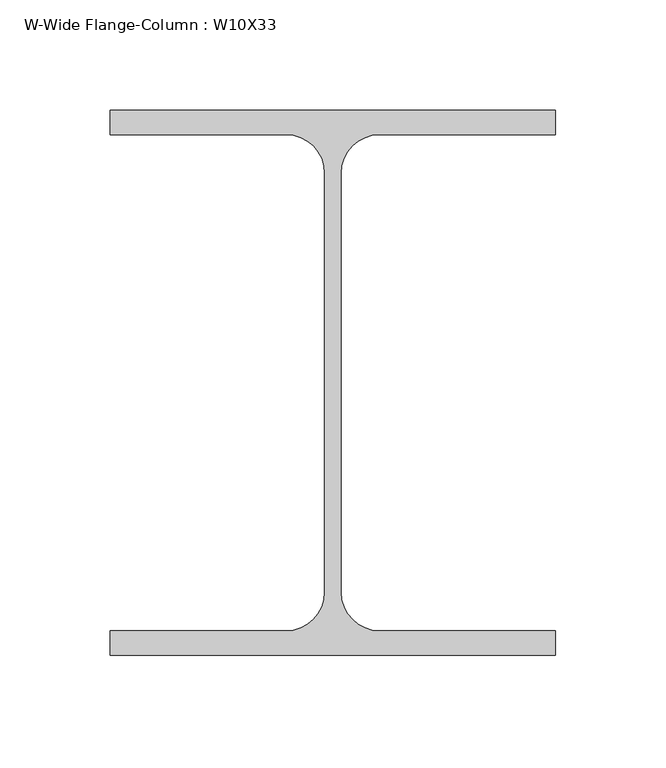
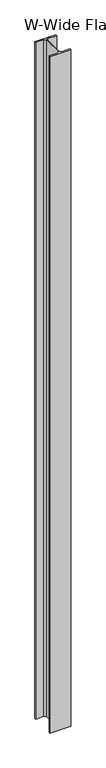
"""IFC4 building model written with IfcOpenShell, lengths in millimetres: column geometry, W-Wide Flange-Column : W10X33."""

from ifc_helpers import new_model, si_unit, point, frame, frame_2d, origin, place, context, project, spatial, polyline, circle_curve, trimmed, segment, composite_curve, outline, extrude, source, transform, mapped, element, save


def w_wide_flange_column_w10x33_8004a937(model_context):
    return source(origin(), model_context, "Body", "SweptSolid", [
        extrude(outline(composite_curve([segment(polyline([(101.092, 123.571), (101.092, 112.522), (21.209, 112.522)]), True, "CONTINUOUS"), segment(trimmed(circle_curve(frame_2d((21.209, 94.996)), 17.526), [point((21.209, 112.522))], [point((3.683, 94.996))], True, "CARTESIAN"), True, "CONTINUOUS"), segment(polyline([(3.683, 94.996), (3.683, -94.996)]), True, "CONTINUOUS"), segment(trimmed(circle_curve(frame_2d((21.209, -94.996)), 17.526), [point((3.683, -94.996))], [point((21.209, -112.522))], True, "CARTESIAN"), True, "CONTINUOUS"), segment(polyline([(21.209, -112.522), (101.092, -112.522), (101.092, -123.571), (-101.092, -123.571), (-101.092, -112.522), (-21.209, -112.522)]), True, "CONTINUOUS"), segment(trimmed(circle_curve(frame_2d((-21.209, -94.996)), 17.526), [point((-21.209, -112.522))], [point((-3.683, -94.996))], True, "CARTESIAN"), True, "CONTINUOUS"), segment(polyline([(-3.683, -94.996), (-3.683, 94.996)]), True, "CONTINUOUS"), segment(trimmed(circle_curve(frame_2d((-21.209, 94.996)), 17.526), [point((-3.683, 94.996))], [point((-21.209, 112.522))], True, "CARTESIAN"), True, "CONTINUOUS"), segment(polyline([(-21.209, 112.522), (-101.092, 112.522), (-101.092, 123.571), (101.092, 123.571)]), True, "CONTINUOUS")], self_intersect=False)), frame((0.0, 0.0, 16408.4), z_axis=(0.0, 0.0, 1.0), x_axis=(1.0, 0.0, 0.0)), (0.0, 0.0, 1.0), 6908.8),
    ])


if __name__ == "__main__":
    model = new_model("IFC4")
    model_context = context("Model", 3, world=origin())
    ifc_project = project(units=[si_unit("LENGTHUNIT", "METRE", prefix="MILLI")], contexts=[model_context])
    site = spatial("IfcSite", under=ifc_project)
    building = spatial("IfcBuilding", under=site)
    placement = place(None, origin())
    w_wide_flange_column_w10x33_shape = w_wide_flange_column_w10x33_8004a937(model_context)
    element("IfcColumn", 1, ObjectType="W-Wide Flange-Column : W10X33", at=placement, inside=building, context=model_context, shape_type="MappedRepresentation", body=[
        mapped(w_wide_flange_column_w10x33_shape, transform((0.0, 0.0, 0.0), x_axis=(1.0, 0.0, 0.0), y_axis=(0.0, 1.0, 0.0), z_axis=(0.0, 0.0, 1.0))),
    ])
    save(model, "model.ifc")

# Revit data of these elements
# Type "W-Wide Flange-Column : W10X33"
#   Assembly Code = "B10"
#   W = 33
#   bf = 0' - 7.96"
#   d = 0' - 9.73"
#   k = 0' - 1 1/8"
#   kr = 0' - 0.69"
#   tf = 0' - 0.435"
#   tw = 0' - 0.29"
#   A = 0.0674306 SF
#   Structural Material [instance default] = Steel ASTM A992
# Element 1 (IfcColumn, "W-Wide Flange-Column : W10X33")
#   Materials on its faces: "Steel ASTM A992"
# Materials
#   "Steel ASTM A992": class "Metal", colour RGB 199 199 199, transparency 0, Description = "Structural steel 50ksi", Cost = 0
